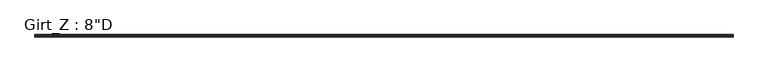
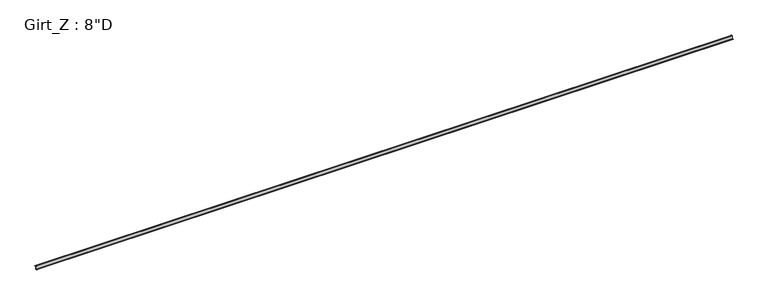
"""IFC4 building model written with IfcOpenShell, lengths in millimetres: beam geometry."""

from ifc_helpers import new_model, si_unit, point, frame, frame_2d, origin, place, context, project, spatial, polyline, circle_curve, trimmed, segment, composite_curve, outline, extrude, source, transform, mapped, element, save


def beam_9cdb4bda(model_context):
    return source(origin(), model_context, "Body", "SweptSolid", [
        extrude(outline(composite_curve([segment(polyline([(63.5, 101.6), (75.745104, 87.0068534), (73.6169367, 85.221109), (62.204539, 98.821875), (3.3005807, 98.821875)]), True, "CONTINUOUS"), segment(trimmed(circle_curve(frame_2d((3.3741066, 96.8381931)), 1.9850441), [point((3.3005807, 98.821875))], [point((1.3890625, 96.8381931))], True, "CARTESIAN"), True, "CONTINUOUS"), segment(polyline([(1.3890625, 96.8381931), (1.3890625, -96.8375)]), True, "CONTINUOUS"), segment(trimmed(circle_curve(frame_2d((-3.3734375, -96.8375)), 4.7625), [point((1.3890625, -96.8375))], [point((-3.3734375, -101.6))], False, "CARTESIAN"), True, "CONTINUOUS"), segment(polyline([(-3.3734375, -101.6), (-63.5, -101.6), (-75.745104, -87.0068534), (-73.6169367, -85.221109), (-62.204539, -98.821875), (-3.2694106, -98.821875)]), True, "CONTINUOUS"), segment(trimmed(circle_curve(frame_2d((-3.3748024, -96.8389339)), 1.9857399), [point((-3.2694106, -98.821875))], [point((-1.3890625, -96.8389339))], True, "CARTESIAN"), True, "CONTINUOUS"), segment(polyline([(-1.3890625, -96.8389339), (-1.3890625, 96.8375)]), True, "CONTINUOUS"), segment(trimmed(circle_curve(frame_2d((3.3734375, 96.8375)), 4.7625), [point((-1.3890625, 96.8375))], [point((3.3734375, 101.6))], False, "CARTESIAN"), True, "CONTINUOUS"), segment(polyline([(3.3734375, 101.6), (63.5, 101.6)]), True, "CONTINUOUS")], self_intersect=False)), frame((-22028.15, 0.0, 0.0), z_axis=(1.0, 0.0, 0.0), x_axis=(0.0, 1.0, 0.0)), (0.0, 0.0, 1.0), 44056.3),
    ])


if __name__ == "__main__":
    model = new_model("IFC4")
    model_context = context("Model", 3, world=origin())
    ifc_project = project(units=[si_unit("LENGTHUNIT", "METRE", prefix="MILLI")], contexts=[model_context])
    site = spatial("IfcSite", under=ifc_project)
    building = spatial("IfcBuilding", under=site)
    placement = place(None, origin())
    beam_shape = beam_9cdb4bda(model_context)
    element("IfcBeam", 1, ObjectType="Girt_Z : 8\"D", at=placement, inside=building, context=model_context, shape_type="MappedRepresentation", body=[
        mapped(beam_shape, transform((0.0, 0.0, 0.0), x_axis=(1.0, 0.0, 0.0), y_axis=(0.0, 1.0, 0.0), z_axis=(0.0, 0.0, 1.0))),
    ])
    save(model, "model.ifc")

# Revit data of these elements
# Type "Girt_Z : 8\"D"
#   Web_Thickness = 0' - 0 7/64"
#   Length [instance default] = 10' - 0"
#   Leg_1 = 0' - 2 1/2"
#   Height = 0' - 8"
#   Structural Material [instance default] = none
